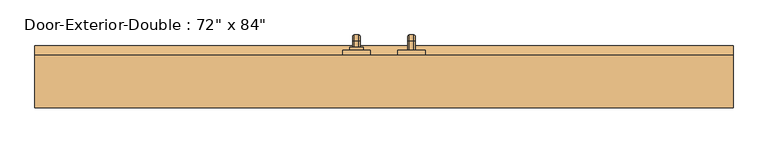
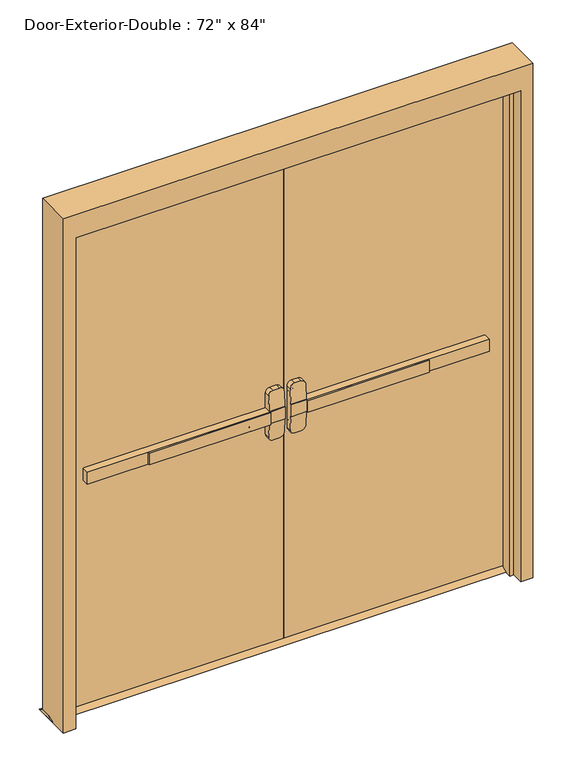
"""IFC4 building model written with IfcOpenShell, lengths in millimetres: door geometry."""

from ifc_helpers import new_model, si_unit, point, frame, frame_2d, origin, place, context, project, spatial, polyline, circle_curve, ellipse_curve, trimmed, segment, composite_curve, outline, extrude, faceted_brep, source, transform, mapped, element, save
from ifc_brep_helpers import plane_surface, cylinder_surface, revolved_surface, advanced_brep


def door_9270c923(model_context):
    return source(origin(), model_context, "Body", "SolidModel", [
        extrude(outline(polyline([(-575.7333333, -25.4), (-575.7333333, -19.05), (-76.2, -19.05), (-76.2, -25.4), (-575.7333333, -25.4)])), frame((0.0, 0.0, 990.6), z_axis=(0.0, 0.0, 1.0), x_axis=(1.0, 0.0, 0.0)), (0.0, 0.0, 1.0), 50.8),
        advanced_brep(
        [(-12.7, -19.05, 1041.4), (-76.2, -19.05, 1041.4), (-825.5, -19.05, 1041.4), (-825.5, -19.05, 990.6), (-76.2, -19.05, 990.6), (-12.7, -19.05, 990.6), (-825.5, 12.7, 1041.4), (-76.2, 12.7, 1041.4), (-76.2, 12.7, 1104.9), (-57.15, 12.7, 1123.95), (-31.75, 12.7, 1123.95), (-12.7, 12.7, 1104.9), (-12.7, 12.7, 927.1), (-31.75, 12.7, 908.05), (-57.15, 12.7, 908.05), (-76.2, 12.7, 927.1), (-76.2, 12.7, 990.6), (-825.5, 12.7, 990.6), (-12.7, -15.8747533, 1041.4), (-76.2, -15.8747533, 1041.4), (-12.7, -15.8747533, 990.6), (-12.7, -10.8645731, 927.1), (-12.7, -10.8645731, 1104.9), (-76.2, -15.8747533, 990.6), (-76.2, -10.8645731, 1104.9), (-76.2, -10.8645731, 927.1), (-57.15, -9.361519, 1123.95), (-31.75, -9.361519, 1123.95), (-31.75, -9.361519, 908.05), (-57.15, -9.361519, 908.05)],
        [
            (0, 1),
            (1, 2),
            (2, 3),
            (3, 4),
            (4, 5),
            (5, 0),
            (6, 7),
            (7, 8),
            (8, 9, circle_curve(frame((-57.15, 12.7, 1104.9), z_axis=(0.0, 1.0, 0.0), x_axis=(-1.0, 0.0, 0.0)), 19.05)),
            (9, 10),
            (10, 11, circle_curve(frame((-31.75, 12.7, 1104.9), z_axis=(0.0, 1.0, 0.0), x_axis=(-1.0, 0.0, 0.0)), 19.05)),
            (11, 12),
            (12, 13, circle_curve(frame((-31.75, 12.7, 927.1), z_axis=(0.0, 1.0, 0.0), x_axis=(-1.0, 0.0, 0.0)), 19.05)),
            (13, 14),
            (14, 15, circle_curve(frame((-57.15, 12.7, 927.1), z_axis=(0.0, 1.0, 0.0), x_axis=(-1.0, 0.0, 0.0)), 19.05)),
            (15, 16),
            (16, 17),
            (17, 6),
            (0, 18),
            (18, 19),
            (19, 7),
            (6, 2),
            (5, 20),
            (20, 21),
            (21, 12),
            (11, 22),
            (22, 18),
            (16, 23),
            (23, 20),
            (3, 17),
            (19, 24),
            (24, 8),
            (15, 25),
            (25, 23),
            (9, 26),
            (26, 27),
            (27, 10),
            (13, 28),
            (28, 29),
            (29, 14),
            (29, 25, ellipse_curve(frame((-57.15, -10.8645731, 927.1), z_axis=(0.0, 0.9969018152893365, 0.07865602756830282), x_axis=(0.0, -0.07865602756830208, 0.9969018152893365)), 19.1092038, 19.05)),
            (24, 26, ellipse_curve(frame((-57.15, -10.8645731, 1104.9), z_axis=(0.0, 0.9969018152893376, -0.07865602756828934), x_axis=(0.0, -0.078656027568288, -0.9969018152893377)), 19.1092038, 19.05)),
            (27, 22, ellipse_curve(frame((-31.75, -10.8645731, 1104.9), z_axis=(0.0, 0.9969018152893376, -0.07865602756828934), x_axis=(0.0, -0.078656027568288, -0.9969018152893377)), 19.1092038, 19.05)),
            (21, 28, ellipse_curve(frame((-31.75, -10.8645731, 927.1), z_axis=(0.0, 0.9969018152893365, 0.07865602756830282), x_axis=(0.0, -0.07865602756830208, 0.9969018152893365)), 19.1092038, 19.05)),
        ],
        [
            plane_surface(frame((-12.7, -19.05, 1041.4), z_axis=(0.0, -1.0, 0.0), x_axis=(1.0, 0.0, 0.0))),
            plane_surface(frame((-12.7, 12.7, 1041.4), z_axis=(0.0, 1.0, 0.0), x_axis=(-1.0, 0.0, 0.0))),
            plane_surface(frame((-825.5, -19.05, 1041.4), z_axis=(0.0, 0.0, 1.0), x_axis=(0.0, 1.0, 0.0))),
            plane_surface(frame((-12.7, -19.05, 1041.4), z_axis=(1.0, 0.0, 0.0), x_axis=(0.0, 1.0, 0.0))),
            plane_surface(frame((-12.7, -19.05, 990.6), z_axis=(0.0, 0.0, -1.0), x_axis=(0.0, 1.0, 0.0))),
            plane_surface(frame((-825.5, -19.05, 990.6), z_axis=(-1.0, 0.0, 0.0), x_axis=(0.0, 1.0, 0.0))),
            plane_surface(frame((-76.2, -15.8747533, 927.1), z_axis=(-1.0, 0.0, 0.0), x_axis=(0.0, 1.0, 0.0))),
            plane_surface(frame((-57.15, -15.8747533, 1123.95), z_axis=(0.0, 0.0, 1.0), x_axis=(0.0, 1.0, 0.0))),
            plane_surface(frame((-31.75, -15.8747533, 908.05), z_axis=(0.0, 0.0, -1.0), x_axis=(0.0, 1.0, 0.0))),
            cylinder_surface(frame((-57.15, 12.7, 927.1), z_axis=(0.0, -1.0, 0.0), x_axis=(-1.0, 0.0, 0.0)), 19.05),
            cylinder_surface(frame((-57.15, 12.7, 1104.9), z_axis=(0.0, -1.0, 0.0), x_axis=(-1.0, 0.0, 0.0)), 19.05),
            cylinder_surface(frame((-31.75, 12.7, 1104.9), z_axis=(0.0, -1.0, 0.0), x_axis=(-1.0, 0.0, 0.0)), 19.05),
            cylinder_surface(frame((-31.75, 12.7, 927.1), z_axis=(0.0, -1.0, 0.0), x_axis=(-1.0, 0.0, 0.0)), 19.05),
            plane_surface(frame((-76.2, -15.8747533, 1041.4), z_axis=(0.0, -0.9969018152893376, 0.07865602756828934), x_axis=(1.0, 0.0, 0.0))),
            plane_surface(frame((-76.2, -9.361519, 908.05), z_axis=(0.0, -0.9969018152893365, -0.07865602756830282), x_axis=(1.0, 0.0, 0.0))),
        ],
        [
            (0, [[1, 2, 3, 4, 5, 6]]),
            (1, [[7, 8, 9, 10, 11, 12, 13, 14, 15, 16, 17, 18]]),
            (2, [[-2, -1, 19, 20, 21, -7, 22]]),
            (3, [[23, 24, 25, -12, 26, 27, -19, -6]]),
            (4, [[-17, 28, 29, -23, -5, -4, 30]]),
            (5, [[-22, -18, -30, -3]]),
            (6, [[-21, 31, 32, -8]]),
            (6, [[33, 34, -28, -16]]),
            (7, [[35, 36, 37, -10]]),
            (8, [[38, 39, 40, -14]]),
            (9, [[-40, 41, -33, -15]]),
            (10, [[-32, 42, -35, -9]]),
            (11, [[-37, 43, -26, -11]]),
            (12, [[-25, 44, -38, -13]]),
            (13, [[-27, -43, -36, -42, -31, -20]]),
            (14, [[-29, -34, -41, -39, -44, -24]]),
        ],
    ),
        extrude(outline(polyline([(57.15, 12.7), (82.55, 0.0), (-12.7, 0.0), (12.7, 12.7), (57.15, 12.7)])), frame((-965.2, 0.0, 0.0), z_axis=(1.0, 0.0, 0.0), x_axis=(0.0, 1.0, 0.0)), (0.0, 0.0, 1.0), 1930.4),
        extrude(outline(polyline([(575.7333333, -25.4), (76.2, -25.4), (76.2, -19.05), (575.7333333, -19.05), (575.7333333, -25.4)])), frame((0.0, 0.0, 990.6), z_axis=(0.0, 0.0, 1.0), x_axis=(1.0, 0.0, 0.0)), (0.0, 0.0, 1.0), 50.8),
        advanced_brep(
        [(12.7, -19.05, 1041.4), (12.7, -19.05, 990.6), (76.2, -19.05, 990.6), (825.5, -19.05, 990.6), (825.5, -19.05, 1041.4), (76.2, -19.05, 1041.4), (825.5, 12.7, 1041.4), (825.5, 12.7, 990.6), (76.2, 12.7, 990.6), (76.2, 12.7, 927.1), (57.15, 12.7, 908.05), (31.75, 12.7, 908.05), (12.7, 12.7, 927.1), (12.7, 12.7, 1104.9), (31.75, 12.7, 1123.95), (57.15, 12.7, 1123.95), (76.2, 12.7, 1104.9), (76.2, 12.7, 1041.4), (76.2, -15.8747533, 1041.4), (12.7, -15.8747533, 1041.4), (12.7, -10.8645731, 1104.9), (12.7, -10.8645731, 927.1), (12.7, -15.8747533, 990.6), (76.2, -15.8747533, 990.6), (76.2, -10.8645731, 927.1), (76.2, -10.8645731, 1104.9), (31.75, -9.361519, 1123.95), (57.15, -9.361519, 1123.95), (57.15, -9.361519, 908.05), (31.75, -9.361519, 908.05)],
        [
            (0, 1),
            (1, 2),
            (2, 3),
            (3, 4),
            (4, 5),
            (5, 0),
            (6, 7),
            (7, 8),
            (8, 9),
            (9, 10, circle_curve(frame((57.15, 12.7, 927.1), z_axis=(0.0, 1.0, 0.0), x_axis=(1.0, 0.0, 0.0)), 19.05)),
            (10, 11),
            (11, 12, circle_curve(frame((31.75, 12.7, 927.1), z_axis=(0.0, 1.0, 0.0), x_axis=(1.0, 0.0, 0.0)), 19.05)),
            (12, 13),
            (13, 14, circle_curve(frame((31.75, 12.7, 1104.9), z_axis=(0.0, 1.0, 0.0), x_axis=(1.0, 0.0, 0.0)), 19.05)),
            (14, 15),
            (15, 16, circle_curve(frame((57.15, 12.7, 1104.9), z_axis=(0.0, 1.0, 0.0), x_axis=(1.0, 0.0, 0.0)), 19.05)),
            (16, 17),
            (17, 6),
            (4, 6),
            (17, 18),
            (18, 19),
            (19, 0),
            (19, 20),
            (20, 13),
            (12, 21),
            (21, 22),
            (22, 1),
            (7, 3),
            (22, 23),
            (23, 8),
            (23, 24),
            (24, 9),
            (16, 25),
            (25, 18),
            (14, 26),
            (26, 27),
            (27, 15),
            (10, 28),
            (28, 29),
            (29, 11),
            (24, 28, ellipse_curve(frame((57.15, -10.8645731, 927.1), z_axis=(0.0, 0.9969018152893365, 0.07865602756830282), x_axis=(0.0, -0.07865602756830208, 0.9969018152893365)), 19.1092038, 19.05)),
            (27, 25, ellipse_curve(frame((57.15, -10.8645731, 1104.9), z_axis=(0.0, 0.9969018152893376, -0.07865602756828934), x_axis=(0.0, -0.078656027568288, -0.9969018152893377)), 19.1092038, 19.05)),
            (20, 26, ellipse_curve(frame((31.75, -10.8645731, 1104.9), z_axis=(0.0, 0.9969018152893376, -0.07865602756828934), x_axis=(0.0, -0.078656027568288, -0.9969018152893377)), 19.1092038, 19.05)),
            (29, 21, ellipse_curve(frame((31.75, -10.8645731, 927.1), z_axis=(0.0, 0.9969018152893365, 0.07865602756830282), x_axis=(0.0, -0.07865602756830208, 0.9969018152893365)), 19.1092038, 19.05)),
        ],
        [
            plane_surface(frame((12.7, -19.05, 1041.4), z_axis=(0.0, -1.0, 0.0), x_axis=(-1.0, 0.0, 0.0))),
            plane_surface(frame((12.7, 12.7, 1041.4), z_axis=(0.0, 1.0, 0.0), x_axis=(1.0, 0.0, 0.0))),
            plane_surface(frame((825.5, -19.05, 1041.4), z_axis=(0.0, 0.0, 1.0), x_axis=(0.0, 1.0, 0.0))),
            plane_surface(frame((12.7, -19.05, 1041.4), z_axis=(-1.0, 0.0, 0.0), x_axis=(0.0, 1.0, 0.0))),
            plane_surface(frame((12.7, -19.05, 990.6), z_axis=(0.0, 0.0, -1.0), x_axis=(0.0, 1.0, 0.0))),
            plane_surface(frame((825.5, -19.05, 990.6), z_axis=(1.0, 0.0, 0.0), x_axis=(0.0, 1.0, 0.0))),
            plane_surface(frame((76.2, -15.8747533, 927.1), z_axis=(1.0, 0.0, 0.0), x_axis=(0.0, 1.0, 0.0))),
            plane_surface(frame((57.15, -15.8747533, 1123.95), z_axis=(0.0, 0.0, 1.0), x_axis=(0.0, 1.0, 0.0))),
            plane_surface(frame((31.75, -15.8747533, 908.05), z_axis=(0.0, 0.0, -1.0), x_axis=(0.0, 1.0, 0.0))),
            cylinder_surface(frame((57.15, 12.7, 927.1), z_axis=(0.0, -1.0, 0.0), x_axis=(1.0, 0.0, 0.0)), 19.05),
            cylinder_surface(frame((57.15, 12.7, 1104.9), z_axis=(0.0, -1.0, 0.0), x_axis=(1.0, 0.0, 0.0)), 19.05),
            cylinder_surface(frame((31.75, 12.7, 1104.9), z_axis=(0.0, -1.0, 0.0), x_axis=(1.0, 0.0, 0.0)), 19.05),
            cylinder_surface(frame((31.75, 12.7, 927.1), z_axis=(0.0, -1.0, 0.0), x_axis=(1.0, 0.0, 0.0)), 19.05),
            plane_surface(frame((76.2, -15.8747533, 1041.4), z_axis=(0.0, -0.9969018152893376, 0.07865602756828934), x_axis=(-1.0, 0.0, 0.0))),
            plane_surface(frame((76.2, -9.361519, 908.05), z_axis=(0.0, -0.9969018152893365, -0.07865602756830282), x_axis=(-1.0, 0.0, 0.0))),
        ],
        [
            (0, [[1, 2, 3, 4, 5, 6]]),
            (1, [[7, 8, 9, 10, 11, 12, 13, 14, 15, 16, 17, 18]]),
            (2, [[19, -18, 20, 21, 22, -6, -5]]),
            (3, [[-1, -22, 23, 24, -13, 25, 26, 27]]),
            (4, [[28, -3, -2, -27, 29, 30, -8]]),
            (5, [[-4, -28, -7, -19]]),
            (6, [[-9, -30, 31, 32]]),
            (6, [[-17, 33, 34, -20]]),
            (7, [[-15, 35, 36, 37]]),
            (8, [[-11, 38, 39, 40]]),
            (9, [[-10, -32, 41, -38]]),
            (10, [[-16, -37, 42, -33]]),
            (11, [[-14, -24, 43, -35]]),
            (12, [[-12, -40, 44, -25]]),
            (13, [[-21, -34, -42, -36, -43, -23]]),
            (14, [[-26, -44, -39, -41, -31, -29]]),
        ],
    ),
        advanced_brep(
        [(66.2, 69.85, 1017.190625), (66.2, 69.85, 1014.809375), (69.771875, 69.85, 1011.2375), (82.6284594, 69.85, 1011.2375), (86.2, 69.85, 1014.8090406), (86.2, 69.85, 1017.190625), (82.628125, 69.85, 1020.7625), (69.771875, 69.85, 1020.7625), (66.2, 69.85, 887.809375), (69.771875, 69.85, 884.2375), (82.628125, 69.85, 884.2375), (86.2, 69.85, 887.809375), (86.2, 69.85, 890.1909594), (82.6284594, 69.85, 893.7625), (69.771875, 69.85, 893.7625), (66.2, 69.85, 890.190625), (66.2, 95.25, 1017.190625), (66.2, 109.140625, 1003.3), (66.2, 109.140625, 901.7), (66.2, 95.25, 887.809375), (66.2, 95.25, 890.190625), (66.2, 106.759375, 901.7), (66.2, 106.759375, 1003.3), (66.2, 95.25, 1014.809375), (69.771875, 95.25, 1011.2375), (82.6284594, 95.25, 1011.2375), (86.2, 95.25, 1014.8090406), (86.2, 106.7590406, 1003.3), (86.2, 106.7590406, 901.7), (86.2, 95.25, 890.1909594), (86.2, 95.25, 887.809375), (86.2, 109.140625, 901.7), (86.2, 109.140625, 1003.3), (86.2, 95.25, 1017.190625), (82.628125, 95.25, 1020.7625), (69.771875, 95.25, 1020.7625), (69.771875, 103.1875, 1003.3), (82.6284594, 103.1875, 1003.3), (82.628125, 112.7125, 1003.3), (69.771875, 112.7125, 1003.3), (69.771875, 103.1875, 901.7), (82.6284594, 103.1875, 901.7), (82.628125, 112.7125, 901.7), (69.771875, 112.7125, 901.7), (69.771875, 95.25, 893.7625), (82.6284594, 95.25, 893.7625), (82.628125, 95.25, 884.2375), (69.771875, 95.25, 884.2375)],
        [
            (0, 1),
            (1, 2, circle_curve(frame((69.771875, 69.85, 1014.809375), z_axis=(0.0, -1.0, 0.0), x_axis=(0.0, 0.0, 1.0)), 3.571875)),
            (2, 3),
            (3, 4, circle_curve(frame((82.6284594, 69.85, 1014.8090406), z_axis=(0.0, -1.0, 0.0), x_axis=(0.0, 0.0, 1.0)), 3.5715406)),
            (4, 5),
            (5, 6, circle_curve(frame((82.628125, 69.85, 1017.190625), z_axis=(0.0, -1.0, 0.0), x_axis=(0.0, 0.0, 1.0)), 3.571875)),
            (6, 7),
            (7, 0, circle_curve(frame((69.771875, 69.85, 1017.190625), z_axis=(0.0, -1.0, 0.0), x_axis=(0.0, 0.0, 1.0)), 3.571875)),
            (8, 9, circle_curve(frame((69.771875, 69.85, 887.809375), z_axis=(0.0, -1.0, 0.0), x_axis=(0.0, 0.0, -1.0)), 3.571875)),
            (9, 10),
            (10, 11, circle_curve(frame((82.628125, 69.85, 887.809375), z_axis=(0.0, -1.0, 0.0), x_axis=(0.0, 0.0, -1.0)), 3.571875)),
            (11, 12),
            (12, 13, circle_curve(frame((82.6284594, 69.85, 890.1909594), z_axis=(0.0, -1.0, 0.0), x_axis=(0.0, 0.0, -1.0)), 3.5715406)),
            (13, 14),
            (14, 15, circle_curve(frame((69.771875, 69.85, 890.190625), z_axis=(0.0, -1.0, 0.0), x_axis=(0.0, 0.0, -1.0)), 3.571875)),
            (15, 8),
            (0, 16),
            (16, 17, circle_curve(frame((66.2, 95.25, 1003.3), z_axis=(-1.0, 0.0, 0.0), x_axis=(0.0, 0.0, 1.0)), 13.890625)),
            (17, 18),
            (18, 19, circle_curve(frame((66.2, 95.25, 901.7), z_axis=(-1.0, 0.0, 0.0), x_axis=(0.0, 1.0, 0.0)), 13.890625)),
            (19, 8),
            (15, 20),
            (20, 21, circle_curve(frame((66.2, 95.25, 901.7), z_axis=(1.0, 0.0, 0.0), x_axis=(0.0, 1.0, 0.0)), 11.509375)),
            (21, 22),
            (22, 23, circle_curve(frame((66.2, 95.25, 1003.3), z_axis=(1.0, 0.0, 0.0), x_axis=(0.0, 0.0, 1.0)), 11.509375)),
            (23, 1),
            (23, 24, circle_curve(frame((69.771875, 95.25, 1014.809375), z_axis=(0.0, -1.0, 0.0), x_axis=(0.0, 0.0, 1.0)), 3.571875)),
            (24, 2),
            (24, 25),
            (25, 3),
            (25, 26, circle_curve(frame((82.6284594, 95.25, 1014.8090406), z_axis=(0.0, -1.0, 0.0), x_axis=(0.0, 0.0, 1.0)), 3.5715406)),
            (26, 4),
            (26, 27, circle_curve(frame((86.2, 95.25, 1003.3), z_axis=(-1.0, 0.0, 0.0), x_axis=(0.0, 0.0, 1.0)), 11.5090406)),
            (27, 28),
            (28, 29, circle_curve(frame((86.2, 95.25, 901.7), z_axis=(-1.0, 0.0, 0.0), x_axis=(0.0, 1.0, 0.0)), 11.5090406)),
            (29, 12),
            (11, 30),
            (30, 31, circle_curve(frame((86.2, 95.25, 901.7), z_axis=(1.0, 0.0, 0.0), x_axis=(0.0, 1.0, 0.0)), 13.890625)),
            (31, 32),
            (32, 33, circle_curve(frame((86.2, 95.25, 1003.3), z_axis=(1.0, 0.0, 0.0), x_axis=(0.0, 0.0, 1.0)), 13.890625)),
            (33, 5),
            (33, 34, circle_curve(frame((82.628125, 95.25, 1017.190625), z_axis=(0.0, -1.0, 0.0), x_axis=(0.0, 0.0, 1.0)), 3.571875)),
            (34, 6),
            (34, 35),
            (35, 7),
            (35, 16, circle_curve(frame((69.771875, 95.25, 1017.190625), z_axis=(0.0, -1.0, 0.0), x_axis=(0.0, 0.0, 1.0)), 3.571875)),
            (36, 24, circle_curve(frame((69.771875, 95.25, 1003.3), z_axis=(1.0, 0.0, 0.0), x_axis=(0.0, 0.0, 1.0)), 7.9375)),
            (22, 36, circle_curve(frame((69.771875, 106.759375, 1003.3), z_axis=(0.0, 0.0, 1.0), x_axis=(0.0, 1.0, 0.0)), 3.571875)),
            (37, 25, circle_curve(frame((82.6284594, 95.25, 1003.3), z_axis=(1.0, 0.0, 0.0), x_axis=(0.0, 0.0, 1.0)), 7.9375)),
            (36, 37),
            (37, 27, circle_curve(frame((82.6284594, 106.7590406, 1003.3), z_axis=(0.0, 0.0, 1.0), x_axis=(0.0, 1.0, 0.0)), 3.5715406)),
            (38, 34, circle_curve(frame((82.628125, 95.25, 1003.3), z_axis=(1.0, 0.0, 0.0), x_axis=(0.0, 0.0, 1.0)), 17.4625)),
            (32, 38, circle_curve(frame((82.628125, 109.140625, 1003.3), z_axis=(0.0, 0.0, 1.0), x_axis=(0.0, 1.0, 0.0)), 3.571875)),
            (39, 35, circle_curve(frame((69.771875, 95.25, 1003.3), z_axis=(1.0, 0.0, 0.0), x_axis=(0.0, 0.0, 1.0)), 17.4625)),
            (38, 39),
            (39, 17, circle_curve(frame((69.771875, 109.140625, 1003.3), z_axis=(0.0, 0.0, 1.0), x_axis=(0.0, 1.0, 0.0)), 3.571875)),
            (21, 40, circle_curve(frame((69.771875, 106.759375, 901.7), z_axis=(0.0, 0.0, 1.0), x_axis=(0.0, 1.0, 0.0)), 3.571875)),
            (40, 36),
            (40, 41),
            (41, 37),
            (41, 28, circle_curve(frame((82.6284594, 106.7590406, 901.7), z_axis=(0.0, 0.0, 1.0), x_axis=(0.0, 1.0, 0.0)), 3.5715406)),
            (31, 42, circle_curve(frame((82.628125, 109.140625, 901.7), z_axis=(0.0, 0.0, 1.0), x_axis=(0.0, 1.0, 0.0)), 3.571875)),
            (42, 38),
            (42, 43),
            (43, 39),
            (43, 18, circle_curve(frame((69.771875, 109.140625, 901.7), z_axis=(0.0, 0.0, 1.0), x_axis=(0.0, 1.0, 0.0)), 3.571875)),
            (44, 40, circle_curve(frame((69.771875, 95.25, 901.7), z_axis=(1.0, 0.0, 0.0), x_axis=(0.0, 1.0, 0.0)), 7.9375)),
            (20, 44, circle_curve(frame((69.771875, 95.25, 890.190625), z_axis=(0.0, 1.0, 0.0), x_axis=(0.0, 0.0, -1.0)), 3.571875)),
            (45, 41, circle_curve(frame((82.6284594, 95.25, 901.7), z_axis=(1.0, 0.0, 0.0), x_axis=(0.0, 1.0, 0.0)), 7.9375)),
            (44, 45),
            (45, 29, circle_curve(frame((82.6284594, 95.25, 890.1909594), z_axis=(0.0, 1.0, 0.0), x_axis=(0.0, 0.0, -1.0)), 3.5715406)),
            (46, 42, circle_curve(frame((82.628125, 95.25, 901.7), z_axis=(1.0, 0.0, 0.0), x_axis=(0.0, 1.0, 0.0)), 17.4625)),
            (30, 46, circle_curve(frame((82.628125, 95.25, 887.809375), z_axis=(0.0, 1.0, 0.0), x_axis=(0.0, 0.0, -1.0)), 3.571875)),
            (47, 43, circle_curve(frame((69.771875, 95.25, 901.7), z_axis=(1.0, 0.0, 0.0), x_axis=(0.0, 1.0, 0.0)), 17.4625)),
            (46, 47),
            (47, 19, circle_curve(frame((69.771875, 95.25, 887.809375), z_axis=(0.0, 1.0, 0.0), x_axis=(0.0, 0.0, -1.0)), 3.571875)),
            (14, 44),
            (13, 45),
            (10, 46),
            (9, 47),
        ],
        [
            plane_surface(frame((76.2, 69.85, 1016.0), z_axis=(0.0, -1.0, 0.0), x_axis=(1.0, 0.0, 0.0))),
            plane_surface(frame((76.2, 69.85, 889.0), z_axis=(0.0, -1.0, 0.0), x_axis=(1.0, 0.0, 0.0))),
            plane_surface(frame((66.2, 69.85, 1017.190625), z_axis=(-1.0, 0.0, 0.0), x_axis=(0.0, 1.0, 0.0))),
            cylinder_surface(frame((69.771875, 69.85, 1014.809375), z_axis=(0.0, -1.0, 0.0), x_axis=(0.0, 0.0, 1.0)), 3.571875),
            plane_surface(frame((69.771875, 69.85, 1011.2375), z_axis=(0.0, 0.0, -1.0), x_axis=(0.0, 1.0, 0.0))),
            cylinder_surface(frame((82.6284594, 69.85, 1014.8090406), z_axis=(0.0, -1.0, 0.0), x_axis=(0.0, 0.0, 1.0)), 3.5715406),
            plane_surface(frame((86.2, 69.85, 1014.8090406), z_axis=(1.0, 0.0, 0.0), x_axis=(0.0, 1.0, 0.0))),
            cylinder_surface(frame((82.628125, 69.85, 1017.190625), z_axis=(0.0, -1.0, 0.0), x_axis=(0.0, 0.0, 1.0)), 3.571875),
            plane_surface(frame((82.628125, 69.85, 1020.7625), z_axis=(0.0, 0.0, 1.0), x_axis=(0.0, 1.0, 0.0))),
            cylinder_surface(frame((69.771875, 69.85, 1017.190625), z_axis=(0.0, -1.0, 0.0), x_axis=(0.0, 0.0, 1.0)), 3.571875),
            revolved_surface(trimmed(ellipse_curve(frame((69.771875, 95.25, 1014.809375), z_axis=(0.0, -1.0, 0.0), x_axis=(0.0, 0.0, 1.0)), 3.571875, 3.571875), [point((66.2, 95.25, 1014.809375))], [point((69.771875, 95.25, 1011.2375))], True, "CARTESIAN"), (76.2, 95.25, 1003.3), (-1.0, 0.0, 0.0)),
            revolved_surface(polyline([(69.771875, 95.25, 1011.2375), (82.6284594, 95.25, 1011.2375)]), (76.2, 95.25, 1003.3), (-1.0, 0.0, 0.0)),
            revolved_surface(trimmed(ellipse_curve(frame((82.6284594, 95.25, 1014.8090406), z_axis=(0.0, -1.0, 0.0), x_axis=(0.0, 0.0, 1.0)), 3.5715406, 3.5715406), [point((82.6284594, 95.25, 1011.2375))], [point((86.2, 95.25, 1014.8090406))], True, "CARTESIAN"), (76.2, 95.25, 1003.3), (-1.0, 0.0, 0.0)),
            revolved_surface(trimmed(ellipse_curve(frame((82.628125, 95.25, 1017.190625), z_axis=(0.0, -1.0, 0.0), x_axis=(0.0, 0.0, 1.0)), 3.571875, 3.571875), [point((86.2, 95.25, 1017.190625))], [point((82.628125, 95.25, 1020.7625))], True, "CARTESIAN"), (76.2, 95.25, 1003.3), (-1.0, 0.0, 0.0)),
            cylinder_surface(frame((76.2, 95.25, 1003.3), z_axis=(-1.0, 0.0, 0.0), x_axis=(0.0, 0.0, 1.0)), 17.4625),
            revolved_surface(trimmed(ellipse_curve(frame((69.771875, 95.25, 1017.190625), z_axis=(0.0, -1.0, 0.0), x_axis=(0.0, 0.0, 1.0)), 3.571875, 3.571875), [point((69.771875, 95.25, 1020.7625))], [point((66.2, 95.25, 1017.190625))], True, "CARTESIAN"), (76.2, 95.25, 1003.3), (-1.0, 0.0, 0.0)),
            cylinder_surface(frame((69.771875, 106.759375, 1003.3), z_axis=(0.0, 0.0, 1.0), x_axis=(0.0, 1.0, 0.0)), 3.571875),
            plane_surface(frame((69.771875, 103.1875, 1003.3), z_axis=(0.0, -1.0, 0.0), x_axis=(0.0, 0.0, -1.0))),
            cylinder_surface(frame((82.6284594, 106.7590406, 1003.3), z_axis=(0.0, 0.0, 1.0), x_axis=(0.0, 1.0, 0.0)), 3.5715406),
            cylinder_surface(frame((82.628125, 109.140625, 1003.3), z_axis=(0.0, 0.0, 1.0), x_axis=(0.0, 1.0, 0.0)), 3.571875),
            plane_surface(frame((82.628125, 112.7125, 1003.3), z_axis=(0.0, 1.0, 0.0), x_axis=(0.0, 0.0, -1.0))),
            cylinder_surface(frame((69.771875, 109.140625, 1003.3), z_axis=(0.0, 0.0, 1.0), x_axis=(0.0, 1.0, 0.0)), 3.571875),
            revolved_surface(trimmed(ellipse_curve(frame((69.771875, 106.759375, 901.7), z_axis=(0.0, 0.0, 1.0), x_axis=(0.0, 1.0, 0.0)), 3.571875, 3.571875), [point((66.2, 106.759375, 901.7))], [point((69.771875, 103.1875, 901.7))], True, "CARTESIAN"), (76.2, 95.25, 901.7), (-1.0, 0.0, 0.0)),
            revolved_surface(polyline([(69.771875, 103.1875, 901.7), (82.6284594, 103.1875, 901.7)]), (76.2, 95.25, 901.7), (-1.0, 0.0, 0.0)),
            revolved_surface(trimmed(ellipse_curve(frame((82.6284594, 106.7590406, 901.7), z_axis=(0.0, 0.0, 1.0), x_axis=(0.0, 1.0, 0.0)), 3.5715406, 3.5715406), [point((82.6284594, 103.1875, 901.7))], [point((86.2, 106.7590406, 901.7))], True, "CARTESIAN"), (76.2, 95.25, 901.7), (-1.0, 0.0, 0.0)),
            revolved_surface(trimmed(ellipse_curve(frame((82.628125, 109.140625, 901.7), z_axis=(0.0, 0.0, 1.0), x_axis=(0.0, 1.0, 0.0)), 3.571875, 3.571875), [point((86.2, 109.140625, 901.7))], [point((82.628125, 112.7125, 901.7))], True, "CARTESIAN"), (76.2, 95.25, 901.7), (-1.0, 0.0, 0.0)),
            cylinder_surface(frame((76.2, 95.25, 901.7), z_axis=(-1.0, 0.0, 0.0), x_axis=(0.0, 1.0, 0.0)), 17.4625),
            revolved_surface(trimmed(ellipse_curve(frame((69.771875, 109.140625, 901.7), z_axis=(0.0, 0.0, 1.0), x_axis=(0.0, 1.0, 0.0)), 3.571875, 3.571875), [point((69.771875, 112.7125, 901.7))], [point((66.2, 109.140625, 901.7))], True, "CARTESIAN"), (76.2, 95.25, 901.7), (-1.0, 0.0, 0.0)),
            cylinder_surface(frame((69.771875, 95.25, 890.190625), z_axis=(0.0, 1.0, 0.0), x_axis=(0.0, 0.0, -1.0)), 3.571875),
            plane_surface(frame((69.771875, 95.25, 893.7625), z_axis=(0.0, 0.0, 1.0), x_axis=(0.0, -1.0, 0.0))),
            cylinder_surface(frame((82.6284594, 95.25, 890.1909594), z_axis=(0.0, 1.0, 0.0), x_axis=(0.0, 0.0, -1.0)), 3.5715406),
            cylinder_surface(frame((82.628125, 95.25, 887.809375), z_axis=(0.0, 1.0, 0.0), x_axis=(0.0, 0.0, -1.0)), 3.571875),
            plane_surface(frame((82.628125, 95.25, 884.2375), z_axis=(0.0, 0.0, -1.0), x_axis=(0.0, -1.0, 0.0))),
            cylinder_surface(frame((69.771875, 95.25, 887.809375), z_axis=(0.0, 1.0, 0.0), x_axis=(0.0, 0.0, -1.0)), 3.571875),
        ],
        [
            (0, [[1, 2, 3, 4, 5, 6, 7, 8]]),
            (1, [[9, 10, 11, 12, 13, 14, 15, 16]]),
            (2, [[-1, 17, 18, 19, 20, 21, -16, 22, 23, 24, 25, 26]]),
            (3, [[-2, -26, 27, 28]]),
            (4, [[-3, -28, 29, 30]]),
            (5, [[-4, -30, 31, 32]]),
            (6, [[-5, -32, 33, 34, 35, 36, -12, 37, 38, 39, 40, 41]]),
            (7, [[-6, -41, 42, 43]]),
            (8, [[-7, -43, 44, 45]]),
            (9, [[-8, -45, 46, -17]]),
            (10, [[47, -27, -25, 48]]),
            (11, [[49, -29, -47, 50]]),
            (12, [[-33, -31, -49, 51]]),
            (13, [[52, -42, -40, 53]]),
            (14, [[54, -44, -52, 55]]),
            (15, [[-18, -46, -54, 56]]),
            (16, [[-48, -24, 57, 58]]),
            (17, [[-50, -58, 59, 60]]),
            (18, [[-51, -60, 61, -34]]),
            (19, [[-53, -39, 62, 63]]),
            (20, [[-55, -63, 64, 65]]),
            (21, [[-56, -65, 66, -19]]),
            (22, [[67, -57, -23, 68]]),
            (23, [[69, -59, -67, 70]]),
            (24, [[-35, -61, -69, 71]]),
            (25, [[72, -62, -38, 73]]),
            (26, [[74, -64, -72, 75]]),
            (27, [[-20, -66, -74, 76]]),
            (28, [[-68, -22, -15, 77]]),
            (29, [[-70, -77, -14, 78]]),
            (30, [[-71, -78, -13, -36]]),
            (31, [[-73, -37, -11, 79]]),
            (32, [[-75, -79, -10, 80]]),
            (33, [[-76, -80, -9, -21]]),
        ],
    ),
        extrude(outline(composite_curve([segment(trimmed(circle_curve(frame_2d((1113.0338574, 76.2)), 89.3016225), [point((1193.8, 114.3))], [point((1193.8, 38.1))], False, "CARTESIAN"), True, "CONTINUOUS"), segment(polyline([(1193.8, 38.1), (838.2, 38.1)]), True, "CONTINUOUS"), segment(trimmed(circle_curve(frame_2d((918.9661426, 76.2)), 89.3016225), [point((838.2, 38.1))], [point((838.2, 114.3))], False, "CARTESIAN"), True, "CONTINUOUS"), segment(polyline([(838.2, 114.3), (1193.8, 114.3)]), True, "CONTINUOUS")], self_intersect=False)), frame((0.0, 57.15, 0.0), z_axis=(0.0, 1.0, 0.0), x_axis=(0.0, 0.0, 1.0)), (0.0, 0.0, 1.0), 12.7),
        advanced_brep(
        [(-86.2, 69.85, 1017.190625), (-86.2, 69.85, 1014.809375), (-82.628125, 69.85, 1011.2375), (-69.7715406, 69.85, 1011.2375), (-66.2, 69.85, 1014.8090406), (-66.2, 69.85, 1017.190625), (-69.771875, 69.85, 1020.7625), (-82.628125, 69.85, 1020.7625), (-86.2, 69.85, 887.809375), (-82.628125, 69.85, 884.2375), (-69.771875, 69.85, 884.2375), (-66.2, 69.85, 887.809375), (-66.2, 69.85, 890.1909594), (-69.7715406, 69.85, 893.7625), (-82.628125, 69.85, 893.7625), (-86.2, 69.85, 890.190625), (-86.2, 95.25, 1017.190625), (-86.2, 109.140625, 1003.3), (-86.2, 109.140625, 901.7), (-86.2, 95.25, 887.809375), (-86.2, 95.25, 890.190625), (-86.2, 106.759375, 901.7), (-86.2, 106.759375, 1003.3), (-86.2, 95.25, 1014.809375), (-82.628125, 95.25, 1011.2375), (-69.7715406, 95.25, 1011.2375), (-66.2, 95.25, 1014.8090406), (-66.2, 106.7590406, 1003.3), (-66.2, 106.7590406, 901.7), (-66.2, 95.25, 890.1909594), (-66.2, 95.25, 887.809375), (-66.2, 109.140625, 901.7), (-66.2, 109.140625, 1003.3), (-66.2, 95.25, 1017.190625), (-69.771875, 95.25, 1020.7625), (-82.628125, 95.25, 1020.7625), (-82.628125, 103.1875, 1003.3), (-69.7715406, 103.1875, 1003.3), (-69.771875, 112.7125, 1003.3), (-82.628125, 112.7125, 1003.3), (-82.628125, 103.1875, 901.7), (-69.7715406, 103.1875, 901.7), (-69.771875, 112.7125, 901.7), (-82.628125, 112.7125, 901.7), (-82.628125, 95.25, 893.7625), (-69.7715406, 95.25, 893.7625), (-69.771875, 95.25, 884.2375), (-82.628125, 95.25, 884.2375)],
        [
            (0, 1),
            (1, 2, circle_curve(frame((-82.628125, 69.85, 1014.809375), z_axis=(0.0, -1.0, 0.0), x_axis=(0.0, 0.0, 1.0)), 3.571875)),
            (2, 3),
            (3, 4, circle_curve(frame((-69.7715406, 69.85, 1014.8090406), z_axis=(0.0, -1.0, 0.0), x_axis=(0.0, 0.0, 1.0)), 3.5715406)),
            (4, 5),
            (5, 6, circle_curve(frame((-69.771875, 69.85, 1017.190625), z_axis=(0.0, -1.0, 0.0), x_axis=(0.0, 0.0, 1.0)), 3.571875)),
            (6, 7),
            (7, 0, circle_curve(frame((-82.628125, 69.85, 1017.190625), z_axis=(0.0, -1.0, 0.0), x_axis=(0.0, 0.0, 1.0)), 3.571875)),
            (8, 9, circle_curve(frame((-82.628125, 69.85, 887.809375), z_axis=(0.0, -1.0, 0.0), x_axis=(0.0, 0.0, -1.0)), 3.571875)),
            (9, 10),
            (10, 11, circle_curve(frame((-69.771875, 69.85, 887.809375), z_axis=(0.0, -1.0, 0.0), x_axis=(0.0, 0.0, -1.0)), 3.571875)),
            (11, 12),
            (12, 13, circle_curve(frame((-69.7715406, 69.85, 890.1909594), z_axis=(0.0, -1.0, 0.0), x_axis=(0.0, 0.0, -1.0)), 3.5715406)),
            (13, 14),
            (14, 15, circle_curve(frame((-82.628125, 69.85, 890.190625), z_axis=(0.0, -1.0, 0.0), x_axis=(0.0, 0.0, -1.0)), 3.571875)),
            (15, 8),
            (0, 16),
            (16, 17, circle_curve(frame((-86.2, 95.25, 1003.3), z_axis=(-1.0, 0.0, 0.0), x_axis=(0.0, 0.0, 1.0)), 13.890625)),
            (17, 18),
            (18, 19, circle_curve(frame((-86.2, 95.25, 901.7), z_axis=(-1.0, 0.0, 0.0), x_axis=(0.0, 1.0, 0.0)), 13.890625)),
            (19, 8),
            (15, 20),
            (20, 21, circle_curve(frame((-86.2, 95.25, 901.7), z_axis=(1.0, 0.0, 0.0), x_axis=(0.0, 1.0, 0.0)), 11.509375)),
            (21, 22),
            (22, 23, circle_curve(frame((-86.2, 95.25, 1003.3), z_axis=(1.0, 0.0, 0.0), x_axis=(0.0, 0.0, 1.0)), 11.509375)),
            (23, 1),
            (23, 24, circle_curve(frame((-82.628125, 95.25, 1014.809375), z_axis=(0.0, -1.0, 0.0), x_axis=(0.0, 0.0, 1.0)), 3.571875)),
            (24, 2),
            (24, 25),
            (25, 3),
            (25, 26, circle_curve(frame((-69.7715406, 95.25, 1014.8090406), z_axis=(0.0, -1.0, 0.0), x_axis=(0.0, 0.0, 1.0)), 3.5715406)),
            (26, 4),
            (26, 27, circle_curve(frame((-66.2, 95.25, 1003.3), z_axis=(-1.0, 0.0, 0.0), x_axis=(0.0, 0.0, 1.0)), 11.5090406)),
            (27, 28),
            (28, 29, circle_curve(frame((-66.2, 95.25, 901.7), z_axis=(-1.0, 0.0, 0.0), x_axis=(0.0, 1.0, 0.0)), 11.5090406)),
            (29, 12),
            (11, 30),
            (30, 31, circle_curve(frame((-66.2, 95.25, 901.7), z_axis=(1.0, 0.0, 0.0), x_axis=(0.0, 1.0, 0.0)), 13.890625)),
            (31, 32),
            (32, 33, circle_curve(frame((-66.2, 95.25, 1003.3), z_axis=(1.0, 0.0, 0.0), x_axis=(0.0, 0.0, 1.0)), 13.890625)),
            (33, 5),
            (33, 34, circle_curve(frame((-69.771875, 95.25, 1017.190625), z_axis=(0.0, -1.0, 0.0), x_axis=(0.0, 0.0, 1.0)), 3.571875)),
            (34, 6),
            (34, 35),
            (35, 7),
            (35, 16, circle_curve(frame((-82.628125, 95.25, 1017.190625), z_axis=(0.0, -1.0, 0.0), x_axis=(0.0, 0.0, 1.0)), 3.571875)),
            (36, 24, circle_curve(frame((-82.628125, 95.25, 1003.3), z_axis=(1.0, 0.0, 0.0), x_axis=(0.0, 0.0, 1.0)), 7.9375)),
            (22, 36, circle_curve(frame((-82.628125, 106.759375, 1003.3), z_axis=(0.0, 0.0, 1.0), x_axis=(0.0, 1.0, 0.0)), 3.571875)),
            (37, 25, circle_curve(frame((-69.7715406, 95.25, 1003.3), z_axis=(1.0, 0.0, 0.0), x_axis=(0.0, 0.0, 1.0)), 7.9375)),
            (36, 37),
            (37, 27, circle_curve(frame((-69.7715406, 106.7590406, 1003.3), z_axis=(0.0, 0.0, 1.0), x_axis=(0.0, 1.0, 0.0)), 3.5715406)),
            (38, 34, circle_curve(frame((-69.771875, 95.25, 1003.3), z_axis=(1.0, 0.0, 0.0), x_axis=(0.0, 0.0, 1.0)), 17.4625)),
            (32, 38, circle_curve(frame((-69.771875, 109.140625, 1003.3), z_axis=(0.0, 0.0, 1.0), x_axis=(0.0, 1.0, 0.0)), 3.571875)),
            (39, 35, circle_curve(frame((-82.628125, 95.25, 1003.3), z_axis=(1.0, 0.0, 0.0), x_axis=(0.0, 0.0, 1.0)), 17.4625)),
            (38, 39),
            (39, 17, circle_curve(frame((-82.628125, 109.140625, 1003.3), z_axis=(0.0, 0.0, 1.0), x_axis=(0.0, 1.0, 0.0)), 3.571875)),
            (21, 40, circle_curve(frame((-82.628125, 106.759375, 901.7), z_axis=(0.0, 0.0, 1.0), x_axis=(0.0, 1.0, 0.0)), 3.571875)),
            (40, 36),
            (40, 41),
            (41, 37),
            (41, 28, circle_curve(frame((-69.7715406, 106.7590406, 901.7), z_axis=(0.0, 0.0, 1.0), x_axis=(0.0, 1.0, 0.0)), 3.5715406)),
            (31, 42, circle_curve(frame((-69.771875, 109.140625, 901.7), z_axis=(0.0, 0.0, 1.0), x_axis=(0.0, 1.0, 0.0)), 3.571875)),
            (42, 38),
            (42, 43),
            (43, 39),
            (43, 18, circle_curve(frame((-82.628125, 109.140625, 901.7), z_axis=(0.0, 0.0, 1.0), x_axis=(0.0, 1.0, 0.0)), 3.571875)),
            (44, 40, circle_curve(frame((-82.628125, 95.25, 901.7), z_axis=(1.0, 0.0, 0.0), x_axis=(0.0, 1.0, 0.0)), 7.9375)),
            (20, 44, circle_curve(frame((-82.628125, 95.25, 890.190625), z_axis=(0.0, 1.0, 0.0), x_axis=(0.0, 0.0, -1.0)), 3.571875)),
            (45, 41, circle_curve(frame((-69.7715406, 95.25, 901.7), z_axis=(1.0, 0.0, 0.0), x_axis=(0.0, 1.0, 0.0)), 7.9375)),
            (44, 45),
            (45, 29, circle_curve(frame((-69.7715406, 95.25, 890.1909594), z_axis=(0.0, 1.0, 0.0), x_axis=(0.0, 0.0, -1.0)), 3.5715406)),
            (46, 42, circle_curve(frame((-69.771875, 95.25, 901.7), z_axis=(1.0, 0.0, 0.0), x_axis=(0.0, 1.0, 0.0)), 17.4625)),
            (30, 46, circle_curve(frame((-69.771875, 95.25, 887.809375), z_axis=(0.0, 1.0, 0.0), x_axis=(0.0, 0.0, -1.0)), 3.571875)),
            (47, 43, circle_curve(frame((-82.628125, 95.25, 901.7), z_axis=(1.0, 0.0, 0.0), x_axis=(0.0, 1.0, 0.0)), 17.4625)),
            (46, 47),
            (47, 19, circle_curve(frame((-82.628125, 95.25, 887.809375), z_axis=(0.0, 1.0, 0.0), x_axis=(0.0, 0.0, -1.0)), 3.571875)),
            (14, 44),
            (13, 45),
            (10, 46),
            (9, 47),
        ],
        [
            plane_surface(frame((-76.2, 69.85, 1016.0), z_axis=(0.0, -1.0, 0.0), x_axis=(1.0, 0.0, 0.0))),
            plane_surface(frame((-76.2, 69.85, 889.0), z_axis=(0.0, -1.0, 0.0), x_axis=(1.0, 0.0, 0.0))),
            plane_surface(frame((-86.2, 69.85, 1017.190625), z_axis=(-1.0, 0.0, 0.0), x_axis=(0.0, 1.0, 0.0))),
            cylinder_surface(frame((-82.628125, 69.85, 1014.809375), z_axis=(0.0, -1.0, 0.0), x_axis=(0.0, 0.0, 1.0)), 3.571875),
            plane_surface(frame((-82.628125, 69.85, 1011.2375), z_axis=(0.0, 0.0, -1.0), x_axis=(0.0, 1.0, 0.0))),
            cylinder_surface(frame((-69.7715406, 69.85, 1014.8090406), z_axis=(0.0, -1.0, 0.0), x_axis=(0.0, 0.0, 1.0)), 3.5715406),
            plane_surface(frame((-66.2, 69.85, 1014.8090406), z_axis=(1.0, 0.0, 0.0), x_axis=(0.0, 1.0, 0.0))),
            cylinder_surface(frame((-69.771875, 69.85, 1017.190625), z_axis=(0.0, -1.0, 0.0), x_axis=(0.0, 0.0, 1.0)), 3.571875),
            plane_surface(frame((-69.771875, 69.85, 1020.7625), z_axis=(0.0, 0.0, 1.0), x_axis=(0.0, 1.0, 0.0))),
            cylinder_surface(frame((-82.628125, 69.85, 1017.190625), z_axis=(0.0, -1.0, 0.0), x_axis=(0.0, 0.0, 1.0)), 3.571875),
            revolved_surface(trimmed(ellipse_curve(frame((-82.628125, 95.25, 1014.809375), z_axis=(0.0, -1.0, 0.0), x_axis=(0.0, 0.0, 1.0)), 3.571875, 3.571875), [point((-86.2, 95.25, 1014.809375))], [point((-82.628125, 95.25, 1011.2375))], True, "CARTESIAN"), (-76.2, 95.25, 1003.3), (-1.0, 0.0, 0.0)),
            revolved_surface(polyline([(-82.628125, 95.25, 1011.2375), (-69.7715406, 95.25, 1011.2375)]), (-76.2, 95.25, 1003.3), (-1.0, 0.0, 0.0)),
            revolved_surface(trimmed(ellipse_curve(frame((-69.7715406, 95.25, 1014.8090406), z_axis=(0.0, -1.0, 0.0), x_axis=(0.0, 0.0, 1.0)), 3.5715406, 3.5715406), [point((-69.7715406, 95.25, 1011.2375))], [point((-66.2, 95.25, 1014.8090406))], True, "CARTESIAN"), (-76.2, 95.25, 1003.3), (-1.0, 0.0, 0.0)),
            revolved_surface(trimmed(ellipse_curve(frame((-69.771875, 95.25, 1017.190625), z_axis=(0.0, -1.0, 0.0), x_axis=(0.0, 0.0, 1.0)), 3.571875, 3.571875), [point((-66.2, 95.25, 1017.190625))], [point((-69.771875, 95.25, 1020.7625))], True, "CARTESIAN"), (-76.2, 95.25, 1003.3), (-1.0, 0.0, 0.0)),
            cylinder_surface(frame((-76.2, 95.25, 1003.3), z_axis=(-1.0, 0.0, 0.0), x_axis=(0.0, 0.0, 1.0)), 17.4625),
            revolved_surface(trimmed(ellipse_curve(frame((-82.628125, 95.25, 1017.190625), z_axis=(0.0, -1.0, 0.0), x_axis=(0.0, 0.0, 1.0)), 3.571875, 3.571875), [point((-82.628125, 95.25, 1020.7625))], [point((-86.2, 95.25, 1017.190625))], True, "CARTESIAN"), (-76.2, 95.25, 1003.3), (-1.0, 0.0, 0.0)),
            cylinder_surface(frame((-82.628125, 106.759375, 1003.3), z_axis=(0.0, 0.0, 1.0), x_axis=(0.0, 1.0, 0.0)), 3.571875),
            plane_surface(frame((-82.628125, 103.1875, 1003.3), z_axis=(0.0, -1.0, 0.0), x_axis=(0.0, 0.0, -1.0))),
            cylinder_surface(frame((-69.7715406, 106.7590406, 1003.3), z_axis=(0.0, 0.0, 1.0), x_axis=(0.0, 1.0, 0.0)), 3.5715406),
            cylinder_surface(frame((-69.771875, 109.140625, 1003.3), z_axis=(0.0, 0.0, 1.0), x_axis=(0.0, 1.0, 0.0)), 3.571875),
            plane_surface(frame((-69.771875, 112.7125, 1003.3), z_axis=(0.0, 1.0, 0.0), x_axis=(0.0, 0.0, -1.0))),
            cylinder_surface(frame((-82.628125, 109.140625, 1003.3), z_axis=(0.0, 0.0, 1.0), x_axis=(0.0, 1.0, 0.0)), 3.571875),
            revolved_surface(trimmed(ellipse_curve(frame((-82.628125, 106.759375, 901.7), z_axis=(0.0, 0.0, 1.0), x_axis=(0.0, 1.0, 0.0)), 3.571875, 3.571875), [point((-86.2, 106.759375, 901.7))], [point((-82.628125, 103.1875, 901.7))], True, "CARTESIAN"), (-76.2, 95.25, 901.7), (-1.0, 0.0, 0.0)),
            revolved_surface(polyline([(-82.628125, 103.1875, 901.7), (-69.7715406, 103.1875, 901.7)]), (-76.2, 95.25, 901.7), (-1.0, 0.0, 0.0)),
            revolved_surface(trimmed(ellipse_curve(frame((-69.7715406, 106.7590406, 901.7), z_axis=(0.0, 0.0, 1.0), x_axis=(0.0, 1.0, 0.0)), 3.5715406, 3.5715406), [point((-69.7715406, 103.1875, 901.7))], [point((-66.2, 106.7590406, 901.7))], True, "CARTESIAN"), (-76.2, 95.25, 901.7), (-1.0, 0.0, 0.0)),
            revolved_surface(trimmed(ellipse_curve(frame((-69.771875, 109.140625, 901.7), z_axis=(0.0, 0.0, 1.0), x_axis=(0.0, 1.0, 0.0)), 3.571875, 3.571875), [point((-66.2, 109.140625, 901.7))], [point((-69.771875, 112.7125, 901.7))], True, "CARTESIAN"), (-76.2, 95.25, 901.7), (-1.0, 0.0, 0.0)),
            cylinder_surface(frame((-76.2, 95.25, 901.7), z_axis=(-1.0, 0.0, 0.0), x_axis=(0.0, 1.0, 0.0)), 17.4625),
            revolved_surface(trimmed(ellipse_curve(frame((-82.628125, 109.140625, 901.7), z_axis=(0.0, 0.0, 1.0), x_axis=(0.0, 1.0, 0.0)), 3.571875, 3.571875), [point((-82.628125, 112.7125, 901.7))], [point((-86.2, 109.140625, 901.7))], True, "CARTESIAN"), (-76.2, 95.25, 901.7), (-1.0, 0.0, 0.0)),
            cylinder_surface(frame((-82.628125, 95.25, 890.190625), z_axis=(0.0, 1.0, 0.0), x_axis=(0.0, 0.0, -1.0)), 3.571875),
            plane_surface(frame((-82.628125, 95.25, 893.7625), z_axis=(0.0, 0.0, 1.0), x_axis=(0.0, -1.0, 0.0))),
            cylinder_surface(frame((-69.7715406, 95.25, 890.1909594), z_axis=(0.0, 1.0, 0.0), x_axis=(0.0, 0.0, -1.0)), 3.5715406),
            cylinder_surface(frame((-69.771875, 95.25, 887.809375), z_axis=(0.0, 1.0, 0.0), x_axis=(0.0, 0.0, -1.0)), 3.571875),
            plane_surface(frame((-69.771875, 95.25, 884.2375), z_axis=(0.0, 0.0, -1.0), x_axis=(0.0, -1.0, 0.0))),
            cylinder_surface(frame((-82.628125, 95.25, 887.809375), z_axis=(0.0, 1.0, 0.0), x_axis=(0.0, 0.0, -1.0)), 3.571875),
        ],
        [
            (0, [[1, 2, 3, 4, 5, 6, 7, 8]]),
            (1, [[9, 10, 11, 12, 13, 14, 15, 16]]),
            (2, [[-1, 17, 18, 19, 20, 21, -16, 22, 23, 24, 25, 26]]),
            (3, [[-2, -26, 27, 28]]),
            (4, [[-3, -28, 29, 30]]),
            (5, [[-4, -30, 31, 32]]),
            (6, [[-5, -32, 33, 34, 35, 36, -12, 37, 38, 39, 40, 41]]),
            (7, [[-6, -41, 42, 43]]),
            (8, [[-7, -43, 44, 45]]),
            (9, [[-8, -45, 46, -17]]),
            (10, [[47, -27, -25, 48]]),
            (11, [[49, -29, -47, 50]]),
            (12, [[-33, -31, -49, 51]]),
            (13, [[52, -42, -40, 53]]),
            (14, [[54, -44, -52, 55]]),
            (15, [[-18, -46, -54, 56]]),
            (16, [[-48, -24, 57, 58]]),
            (17, [[-50, -58, 59, 60]]),
            (18, [[-51, -60, 61, -34]]),
            (19, [[-53, -39, 62, 63]]),
            (20, [[-55, -63, 64, 65]]),
            (21, [[-56, -65, 66, -19]]),
            (22, [[67, -57, -23, 68]]),
            (23, [[69, -59, -67, 70]]),
            (24, [[-35, -61, -69, 71]]),
            (25, [[72, -62, -38, 73]]),
            (26, [[74, -64, -72, 75]]),
            (27, [[-20, -66, -74, 76]]),
            (28, [[-68, -22, -15, 77]]),
            (29, [[-70, -77, -14, 78]]),
            (30, [[-71, -78, -13, -36]]),
            (31, [[-73, -37, -11, 79]]),
            (32, [[-75, -79, -10, 80]]),
            (33, [[-76, -80, -9, -21]]),
        ],
    ),
        extrude(outline(composite_curve([segment(trimmed(circle_curve(frame_2d((1117.6, -76.2)), 19.0), [point((1117.6, -95.2))], [point((1117.6, -57.2))], False, "CARTESIAN"), True, "CONTINUOUS"), segment(trimmed(circle_curve(frame_2d((1117.6, -76.2)), 19.0), [point((1117.6, -57.2))], [point((1117.6, -95.2))], False, "CARTESIAN"), True, "CONTINUOUS")], self_intersect=False)), frame((0.0, 69.85, 0.0), z_axis=(0.0, 1.0, 0.0), x_axis=(0.0, 0.0, 1.0)), (0.0, 0.0, 1.0), 8.73125),
        extrude(outline(composite_curve([segment(trimmed(circle_curve(frame_2d((1113.0338574, -76.2)), 89.3016225), [point((1193.8, -38.1))], [point((1193.8, -114.3))], False, "CARTESIAN"), True, "CONTINUOUS"), segment(polyline([(1193.8, -114.3), (838.2, -114.3)]), True, "CONTINUOUS"), segment(trimmed(circle_curve(frame_2d((918.9661426, -76.2)), 89.3016225), [point((838.2, -114.3))], [point((838.2, -38.1))], False, "CARTESIAN"), True, "CONTINUOUS"), segment(polyline([(838.2, -38.1), (1193.8, -38.1)]), True, "CONTINUOUS")], self_intersect=False)), frame((0.0, 57.15, 0.0), z_axis=(0.0, 1.0, 0.0), x_axis=(0.0, 0.0, 1.0)), (0.0, 0.0, 1.0), 12.7),
        faceted_brep([(914.4, 7.9375, 0.0), (914.4, 57.15, 0.0), (965.2, 57.15, 0.0), (965.2, -88.9, 0.0), (914.4, -88.9, 0.0), (914.4, -39.6875, 0.0), (898.525, -39.6875, 0.0), (898.525, 7.9375, 0.0), (914.4, 7.9375, 2133.6), (914.4, 57.15, 2133.6), (-914.4, 57.15, 2133.6), (-914.4, 57.15, 0.0), (-965.2, 57.15, 0.0), (-965.2, 57.15, 2235.2), (965.2, 57.15, 2235.2), (965.2, -88.9, 2235.2), (-965.2, -88.9, 2235.2), (-965.2, -88.9, 0.0), (-914.4, -88.9, 0.0), (-914.4, -88.9, 2133.6), (914.4, -88.9, 2133.6), (914.4, -39.6875, 2133.6), (-914.4, -39.6875, 2133.6), (-914.4, -39.6875, 0.0), (-898.525, -39.6875, 0.0), (-898.525, -39.6875, 2117.725), (898.525, -39.6875, 2117.725), (898.525, 7.9375, 2117.725), (-898.525, 7.9375, 2117.725), (-898.525, 7.9375, 0.0), (-914.4, 7.9375, 0.0), (-914.4, 7.9375, 2133.6)], [[[0, 1, 2, 3, 4, 5, 6, 7]], [[1, 0, 8, 9]], [[2, 1, 9, 10, 11, 12, 13, 14]], [[3, 2, 14, 15]], [[4, 3, 15, 16, 17, 18, 19, 20]], [[5, 4, 20, 21]], [[6, 5, 21, 22, 23, 24, 25, 26]], [[7, 6, 26, 27]], [[0, 7, 27, 28, 29, 30, 31, 8]], [[9, 8, 31, 10]], [[20, 19, 22, 21]], [[26, 25, 28, 27]], [[12, 11, 30, 29, 24, 23, 18, 17]], [[11, 10, 31, 30]], [[13, 12, 17, 16]], [[19, 18, 23, 22]], [[25, 24, 29, 28]], [[15, 14, 13, 16]]]),
        extrude(outline(polyline([(914.4, 12.7), (1.5875, 12.7), (1.5875, 57.15), (914.4, 57.15), (914.4, 12.7)])), frame((0.0, 0.0, 12.7), z_axis=(0.0, 0.0, 1.0), x_axis=(1.0, 0.0, 0.0)), (0.0, 0.0, 1.0), 2120.9),
        extrude(outline(polyline([(-1.5875, 12.7), (-914.4, 12.7), (-914.4, 57.15), (-1.5875, 57.15), (-1.5875, 12.7)])), frame((0.0, 0.0, 12.7), z_axis=(0.0, 0.0, 1.0), x_axis=(1.0, 0.0, 0.0)), (0.0, 0.0, 1.0), 2120.9),
    ])


if __name__ == "__main__":
    model = new_model("IFC4")
    model_context = context("Model", 3, world=origin())
    ifc_project = project(units=[si_unit("LENGTHUNIT", "METRE", prefix="MILLI")], contexts=[model_context])
    site = spatial("IfcSite", under=ifc_project)
    building = spatial("IfcBuilding", under=site)
    placement = place(None, origin())
    door_shape = door_9270c923(model_context)
    element("IfcDoor", 1, ObjectType="Door-Exterior-Double : 72\" x 84\"", at=placement, inside=building, context=model_context, shape_type="MappedRepresentation", body=[
        mapped(door_shape, transform((0.0, 0.0, 0.0), x_axis=(1.0, 0.0, 0.0), y_axis=(0.0, 1.0, 0.0), z_axis=(0.0, 0.0, 1.0))),
    ])
    save(model, "model.ifc")

# Revit data of these elements
# Type "Door-Exterior-Double : 72\" x 84\""
#   Type Mark = "11"
#   Assembly Code = "B2030200"
#   Analytic Construction = "Metal"
#   Threshold Length [instance default] = 6' - 4"
#   Threshold Offset [instance default] = 0' - 0 1/2"
#   Thickness = 0' - 1 3/4"
#   Thermal Resistance (R) = 0.270118 (m²·K)/W
#   Swing Angle [instance default] = 90.00°
#   Strike Height = 3' - 4"
#   SinglePanelWidth = 3' - 0"
#   Rough Width [instance default] = 6' - 4"
#   Rough Height [instance default] = 7' - 4"
#   MFOpeningHeight [instance default] = 0' - 4"
#   MFOpeningWidth [instance default] = 0' - 4"
#   Inset Calculate [instance default] = 0' - 4"
#   Masonry Inset [instance default] = 0' - 1"
#   Height = 7' - 0"
#   Width = 6' - 0"
#   Heat Transfer Coefficient (U) = 3.70223 W/(m²·K)
#   Masonry Frame Depth = 0' - 5 3/4"
#   Threshold [instance default] = yes
#   Masonry Frame [instance default] = yes
#   Function = 1
#   Dry Wall Frame [instance default] = no
#   Threshold Material = Cherry
#   Panic Bar Material = Metal - Stainless Steel
#   Panel Material = Metal - Painted - Grey
#   Frame Material = Metal - Painted - Grey
#   Exterior Pull Material = Metal - Stainless Steel
#   Visual Light Transmittance = 0
#   Solar Heat Gain Coefficient = 0
#   Wall Closure = (empty or 0)
# Element 1 (IfcDoor, "Door-Exterior-Double : 72\" x 84\"")
#   Materials on its faces: "Metal - Stainless Steel", "Metal - Painted - Grey", "Cherry"
# Materials
#   "Cherry": class "Wood", colour RGB 154 107 61, transparency 0, Description = "Prunus Serotina", Cost = 0
#   "Metal - Stainless Steel": class "Metal", colour RGB 247 247 247, transparency 0
#   "Metal - Painted - Grey": class "Paint", colour RGB 104 104 104, transparency 0
